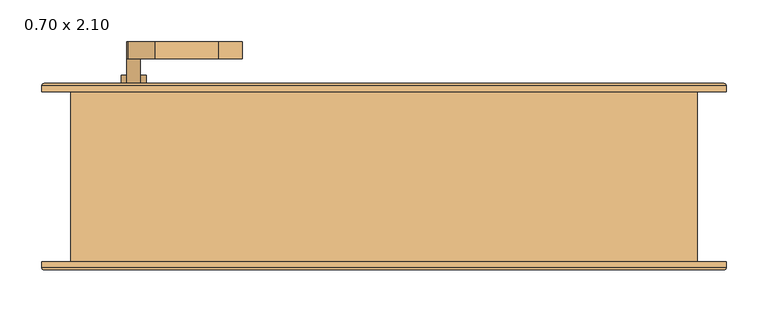
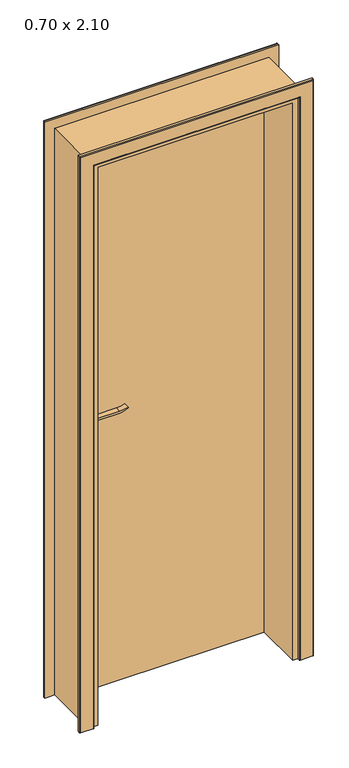
"""IFC4 building model written with IfcOpenShell, lengths in millimetres: door geometry, .CC_ND 300_PORTA SIMPLES DE ABRIR_COM EXTENSÃO : 0.70 x 2.10."""

from ifc_helpers import new_model, si_unit, point, frame, frame_2d, origin, origin_with_axes, place, context, project, spatial, polyline, circle_curve, ellipse_curve, trimmed, segment, composite_curve, outline, extrude, faceted_brep, source, transform, mapped, element, save
from ifc_brep_helpers import plane_surface, cylinder_surface, advanced_brep


def door_0_70_x_2_10_fae9ef36(model_context):
    return source(origin(), model_context, "Body", "SolidModel", [
        extrude(outline(composite_curve([segment(trimmed(circle_curve(frame_2d((964.5, -300.0)), 15.0), [point((964.5, -285.0))], [point((964.5, -315.0))], False, "CARTESIAN"), True, "CONTINUOUS"), segment(trimmed(circle_curve(frame_2d((964.5, -300.0)), 15.0), [point((964.5, -315.0))], [point((964.5, -285.0))], False, "CARTESIAN"), True, "CONTINUOUS")], self_intersect=False)), frame((0.0, 126.4, 0.0), z_axis=(0.0, 1.0, 0.0), x_axis=(0.0, 0.0, 1.0)), (0.0, 0.0, 1.0), 10.0),
        extrude(outline(composite_curve([segment(trimmed(circle_curve(frame_2d((964.5, -300.0)), 15.0), [point((964.5, -285.0))], [point((964.5, -315.0))], False, "CARTESIAN"), True, "CONTINUOUS"), segment(trimmed(circle_curve(frame_2d((964.5, -300.0)), 15.0), [point((964.5, -315.0))], [point((964.5, -285.0))], False, "CARTESIAN"), True, "CONTINUOUS")], self_intersect=False)), frame((0.0, 66.4, 0.0), z_axis=(0.0, 1.0, 0.0), x_axis=(0.0, 0.0, 1.0)), (0.0, 0.0, 1.0), 10.0),
        extrude(outline(composite_curve([segment(trimmed(circle_curve(frame_2d((1024.5, -300.0)), 8.0), [point((1029.1523287, -306.5081363))], [point((1024.5, -292.0))], False, "CARTESIAN"), True, "CONTINUOUS"), segment(trimmed(circle_curve(frame_2d((1019.3738613, -274.6138099)), 18.1261387), [point((1024.5, -292.0))], [point((1037.5, -274.6138099))], True, "CARTESIAN"), True, "CONTINUOUS"), segment(polyline([(1037.5, -274.6138099), (1037.5, -198.3564091)]), True, "CONTINUOUS"), segment(trimmed(circle_curve(frame_2d((1096.7709207, -201.9396612)), 59.3791355), [point((1037.5, -198.3564091))], [point((1046.7135558, -170.0))], False, "CARTESIAN"), True, "CONTINUOUS"), segment(polyline([(1046.7135558, -170.0), (1049.5, -170.0)]), True, "CONTINUOUS"), segment(trimmed(circle_curve(frame_2d((1127.7850638, -198.4227909)), 83.2850902), [point((1049.5, -170.0))], [point((1044.5, -198.3564091))], True, "CARTESIAN"), True, "CONTINUOUS"), segment(polyline([(1044.5, -198.3564091), (1044.5, -274.6325667)]), True, "CONTINUOUS"), segment(trimmed(circle_curve(frame_2d((1007.2555521, -276.3324871)), 37.2832219), [point((1044.5, -274.6325667))], [point((1029.1523287, -306.5081363))], False, "CARTESIAN"), True, "CONTINUOUS")], self_intersect=False)), frame((0.0, 156.4, 0.0), z_axis=(0.0, 1.0, 0.0), x_axis=(0.0, 0.0, 1.0)), (0.0, 0.0, 1.0), 20.0),
        extrude(outline(composite_curve([segment(trimmed(circle_curve(frame_2d((1019.3738682, -274.6138122)), 18.1261318), [point((1024.4999903, -292.0))], [point((1037.5, -274.6138122))], True, "CARTESIAN"), True, "CONTINUOUS"), segment(polyline([(1037.5, -274.6138122), (1037.5, -198.3564091)]), True, "CONTINUOUS"), segment(trimmed(circle_curve(frame_2d((1096.7709207, -201.9396612)), 59.3791355), [point((1037.5, -198.3564091))], [point((1046.7135558, -170.0))], False, "CARTESIAN"), True, "CONTINUOUS"), segment(polyline([(1046.7135558, -170.0), (1049.5, -170.0)]), True, "CONTINUOUS"), segment(trimmed(circle_curve(frame_2d((1127.7850638, -198.4227909)), 83.2850902), [point((1049.5, -170.0))], [point((1044.5, -198.3564091))], True, "CARTESIAN"), True, "CONTINUOUS"), segment(polyline([(1044.5, -198.3564091), (1044.5, -274.6325667)]), True, "CONTINUOUS"), segment(trimmed(circle_curve(frame_2d((1007.2555521, -276.3324871)), 37.2832219), [point((1044.5, -274.6325667))], [point((1029.1523287, -306.5081363))], False, "CARTESIAN"), True, "CONTINUOUS"), segment(trimmed(circle_curve(frame_2d((1024.5, -300.0)), 8.0), [point((1029.1523287, -306.5081363))], [point((1024.4999903, -292.0))], False, "CARTESIAN"), True, "CONTINUOUS")], self_intersect=False)), frame((0.0, 26.4, 0.0), z_axis=(0.0, 1.0, 0.0), x_axis=(0.0, 0.0, 1.0)), (0.0, 0.0, 1.0), 20.0),
        extrude(outline(composite_curve([segment(trimmed(circle_curve(frame_2d((1024.5, -300.0)), 8.0), [point((1024.5, -292.0))], [point((1024.5, -308.0))], False, "CARTESIAN"), True, "CONTINUOUS"), segment(trimmed(circle_curve(frame_2d((1024.5, -300.0)), 8.0), [point((1024.5, -308.0))], [point((1024.5, -292.0))], False, "CARTESIAN"), True, "CONTINUOUS")], self_intersect=False)), frame((0.0, 126.4, 0.0), z_axis=(0.0, 1.0, 0.0), x_axis=(0.0, 0.0, 1.0)), (0.0, 0.0, 1.0), 30.0),
        extrude(outline(composite_curve([segment(trimmed(circle_curve(frame_2d((1024.5, -300.0)), 8.0), [point((1024.5, -292.0))], [point((1024.5, -308.0))], False, "CARTESIAN"), True, "CONTINUOUS"), segment(trimmed(circle_curve(frame_2d((1024.5, -300.0)), 8.0), [point((1024.5, -308.0))], [point((1024.5, -292.0))], False, "CARTESIAN"), True, "CONTINUOUS")], self_intersect=False)), frame((0.0, 46.4, 0.0), z_axis=(0.0, 1.0, 0.0), x_axis=(0.0, 0.0, 1.0)), (0.0, 0.0, 1.0), 30.0),
        extrude(outline(composite_curve([segment(trimmed(circle_curve(frame_2d((954.5, -300.0)), 25.0), [point((954.5, -325.0))], [point((954.5, -275.0))], False, "CARTESIAN"), True, "CONTINUOUS"), segment(polyline([(954.5, -275.0), (1024.5, -275.0)]), True, "CONTINUOUS"), segment(trimmed(circle_curve(frame_2d((1024.5, -300.0)), 25.0), [point((1024.5, -275.0))], [point((1024.5, -325.0))], False, "CARTESIAN"), True, "CONTINUOUS"), segment(polyline([(1024.5, -325.0), (954.5, -325.0)]), True, "CONTINUOUS")], self_intersect=False)), frame((0.0, 116.4, 0.0), z_axis=(0.0, 1.0, 0.0), x_axis=(0.0, 0.0, 1.0)), (0.0, 0.0, 1.0), 10.0),
        extrude(outline(composite_curve([segment(trimmed(circle_curve(frame_2d((954.5, -300.0)), 25.0), [point((954.5, -325.0))], [point((954.5, -275.0))], False, "CARTESIAN"), True, "CONTINUOUS"), segment(polyline([(954.5, -275.0), (1024.5, -275.0)]), True, "CONTINUOUS"), segment(trimmed(circle_curve(frame_2d((1024.5, -300.0)), 25.0), [point((1024.5, -275.0))], [point((1024.5, -325.0))], False, "CARTESIAN"), True, "CONTINUOUS"), segment(polyline([(1024.5, -325.0), (954.5, -325.0)]), True, "CONTINUOUS")], self_intersect=False)), frame((0.0, 76.4, 0.0), z_axis=(0.0, 1.0, 0.0), x_axis=(0.0, 0.0, 1.0)), (0.0, 0.0, 1.0), 10.0),
        faceted_brep([(342.0, -86.9, 0.0), (342.0, 86.4, 0.0), (350.0, 86.4, 0.0), (350.0, 116.4, 0.0), (375.0, 116.4, 0.0), (375.0, -86.9, 0.0), (375.0, -86.9, 2100.0), (-375.0, -86.9, 2100.0), (-375.0, -86.9, 0.0), (-342.0, -86.9, 0.0), (-342.0, -86.9, 2067.0), (342.0, -86.9, 2067.0), (375.0, 116.4, 2100.0), (350.0, 116.4, 2075.0), (-350.0, 116.4, 2075.0), (-350.0, 116.4, 0.0), (-375.0, 116.4, 0.0), (-375.0, 116.4, 2100.0), (350.0, 86.4, 2075.0), (342.0, 86.4, 2067.0), (-342.0, 86.4, 2067.0), (-342.0, 86.4, 0.0), (-350.0, 86.4, 0.0), (-350.0, 86.4, 2075.0)], [[[0, 1, 2, 3, 4, 5]], [[5, 6, 7, 8, 9, 10, 11, 0]], [[4, 12, 6, 5]], [[3, 13, 14, 15, 16, 17, 12, 4]], [[2, 18, 13, 3]], [[1, 19, 20, 21, 22, 23, 18, 2]], [[0, 11, 19, 1]], [[10, 9, 21, 20]], [[9, 8, 16, 15, 22, 21]], [[17, 16, 8, 7]], [[23, 22, 15, 14]], [[12, 17, 7, 6]], [[18, 23, 14, 13]], [[11, 10, 20, 19]]]),
        extrude(outline(polyline([(-350.0, 86.4), (-350.0, 116.4), (350.0, 116.4), (350.0, 86.4), (-350.0, 86.4)])), origin_with_axes(), (0.0, 0.0, 1.0), 2075.0),
        advanced_brep(
        [(-410.0, 116.4, 0.0), (-410.0, 123.4, 0.0), (-407.0, 126.4, 0.0), (-363.0, 126.4, 0.0), (-360.0, 123.4, 0.0), (-360.0, 116.4, 0.0), (-360.0, 116.4, 2085.0), (360.0, 116.4, 2085.0), (360.0, 116.4, 0.0), (410.0, 116.4, 0.0), (410.0, 116.4, 2135.0), (-410.0, 116.4, 2135.0), (-360.0, 123.4, 2085.0), (-363.0, 126.4, 2088.0), (-407.0, 126.4, 2132.0), (407.0, 126.4, 2132.0), (407.0, 126.4, 0.0), (363.0, 126.4, 0.0), (363.0, 126.4, 2088.0), (-410.0, 123.4, 2135.0), (410.0, 123.4, 0.0), (410.0, 123.4, 2135.0), (360.0, 123.4, 0.0), (360.0, 123.4, 2085.0)],
        [
            (0, 1),
            (1, 2, circle_curve(frame((-407.0, 123.4, 0.0), z_axis=(0.0, 0.0, -1.0), x_axis=(1.0, 0.0, 0.0)), 3.0)),
            (2, 3),
            (3, 4, circle_curve(frame((-363.0, 123.4, 0.0), z_axis=(0.0, 0.0, -1.0), x_axis=(1.0, 0.0, 0.0)), 3.0)),
            (4, 5),
            (5, 0),
            (5, 6),
            (6, 7),
            (7, 8),
            (8, 9),
            (9, 10),
            (10, 11),
            (11, 0),
            (4, 12),
            (12, 6),
            (3, 13),
            (13, 12, ellipse_curve(frame((-363.0, 123.4, 2088.0), z_axis=(-0.7071067811865475, 0.0, -0.7071067811865475), x_axis=(0.7071067811865474, 0.0, -0.7071067811865476)), 4.2426407, 3.0)),
            (2, 14),
            (14, 15),
            (15, 16),
            (16, 17),
            (17, 18),
            (18, 13),
            (1, 19),
            (19, 14, ellipse_curve(frame((-407.0, 123.4, 2132.0), z_axis=(-0.7071067811865475, 0.0, -0.7071067811865475), x_axis=(0.7071067811865474, 0.0, -0.7071067811865476)), 4.2426407, 3.0)),
            (11, 19),
            (9, 20),
            (20, 21),
            (21, 10),
            (8, 22),
            (22, 17, circle_curve(frame((363.0, 123.4, 0.0), z_axis=(0.0, 0.0, -1.0), x_axis=(-1.0, 0.0, 0.0)), 3.0)),
            (16, 20, circle_curve(frame((407.0, 123.4, 0.0), z_axis=(0.0, 0.0, -1.0), x_axis=(-1.0, 0.0, 0.0)), 3.0)),
            (23, 22),
            (7, 23),
            (23, 18, ellipse_curve(frame((363.0, 123.4, 2088.0), z_axis=(0.7071067811865475, 0.0, -0.7071067811865475), x_axis=(0.7071067811865474, 0.0, 0.7071067811865476)), 4.2426407, 3.0)),
            (15, 21, ellipse_curve(frame((407.0, 123.4, 2132.0), z_axis=(0.7071067811865475, 0.0, -0.7071067811865475), x_axis=(0.7071067811865474, 0.0, 0.7071067811865476)), 4.2426407, 3.0)),
            (12, 23),
            (21, 19),
        ],
        [
            plane_surface(frame((-360.0, 116.4, 0.0), z_axis=(0.0, 0.0, -1.0), x_axis=(0.0, -1.0, 0.0))),
            plane_surface(frame((-410.0, 116.4, 0.0), z_axis=(0.0, -1.0, 0.0), x_axis=(0.0, 0.0, 1.0))),
            plane_surface(frame((-360.0, 116.4, 0.0), z_axis=(1.0, 0.0, 0.0), x_axis=(0.0, 0.0, 1.0))),
            cylinder_surface(frame((-363.0, 123.4, 0.0), z_axis=(0.0, 0.0, -1.0), x_axis=(1.0, 0.0, 0.0)), 3.0),
            plane_surface(frame((-363.0, 126.4, 0.0), z_axis=(0.0, 1.0, 0.0), x_axis=(0.0, 0.0, 1.0))),
            cylinder_surface(frame((-407.0, 123.4, 0.0), z_axis=(0.0, 0.0, -1.0), x_axis=(1.0, 0.0, 0.0)), 3.0),
            plane_surface(frame((-410.0, 123.4, 0.0), z_axis=(-1.0, 0.0, 0.0), x_axis=(0.0, 0.0, 1.0))),
            plane_surface(frame((410.0, 123.4, 2135.0), z_axis=(1.0, 0.0, 0.0), x_axis=(0.0, 0.0, -1.0))),
            plane_surface(frame((360.0, 116.4, 0.0), z_axis=(0.0, 0.0, -1.0), x_axis=(0.0, -1.0, 0.0))),
            plane_surface(frame((360.0, 116.4, 2085.0), z_axis=(-1.0, 0.0, 0.0), x_axis=(0.0, 0.0, -1.0))),
            cylinder_surface(frame((363.0, 123.4, 2085.0), z_axis=(0.0, 0.0, 1.0), x_axis=(-1.0, 0.0, 0.0)), 3.0),
            cylinder_surface(frame((407.0, 123.4, 2085.0), z_axis=(0.0, 0.0, 1.0), x_axis=(-1.0, 0.0, 0.0)), 3.0),
            plane_surface(frame((-360.0, 116.4, 2085.0), z_axis=(0.0, 0.0, -1.0), x_axis=(1.0, 0.0, 0.0))),
            plane_surface(frame((-410.0, 123.4, 2135.0), z_axis=(0.0, 0.0, 1.0), x_axis=(1.0, 0.0, 0.0))),
            cylinder_surface(frame((-360.0, 123.4, 2088.0), z_axis=(-1.0, 0.0, 0.0), x_axis=(0.0, 0.0, -1.0)), 3.0),
            cylinder_surface(frame((-360.0, 123.4, 2132.0), z_axis=(-1.0, 0.0, 0.0), x_axis=(0.0, 0.0, -1.0)), 3.0),
        ],
        [
            (0, [[1, 2, 3, 4, 5, 6]]),
            (1, [[7, 8, 9, 10, 11, 12, 13, -6]]),
            (2, [[14, 15, -7, -5]]),
            (3, [[16, 17, -14, -4]]),
            (4, [[18, 19, 20, 21, 22, 23, -16, -3]]),
            (5, [[24, 25, -18, -2]]),
            (6, [[-13, 26, -24, -1]]),
            (7, [[-11, 27, 28, 29]]),
            (8, [[-10, 30, 31, -21, 32, -27]]),
            (9, [[33, -30, -9, 34]]),
            (10, [[-22, -31, -33, 35]]),
            (11, [[-28, -32, -20, 36]]),
            (12, [[37, -34, -8, -15]]),
            (13, [[-12, -29, 38, -26]]),
            (14, [[-23, -35, -37, -17]]),
            (15, [[-38, -36, -19, -25]]),
        ],
    ),
        advanced_brep(
        [(410.0, -86.9, 0.0), (410.0, -93.9342217, 0.0), (407.0342217, -96.9, 0.0), (362.9842717, -96.9, 0.0), (360.0, -93.9157283, 0.0), (360.0, -86.9, 0.0), (360.0, -86.9, 2085.0), (-360.0, -86.9, 2085.0), (-360.0, -86.9, 0.0), (-410.0, -86.9, 0.0), (-410.0, -86.9, 2135.0), (410.0, -86.9, 2135.0), (360.0, -93.9157283, 2085.0), (362.9842717, -96.9, 2087.9842717), (407.0342217, -96.9, 2132.0342217), (-407.0342217, -96.9, 2132.0342217), (-407.0342217, -96.9, 0.0), (-362.9842717, -96.9, 0.0), (-362.9842717, -96.9, 2087.9842717), (410.0, -93.9342217, 2135.0), (-410.0, -93.9342217, 0.0), (-410.0, -93.9342217, 2135.0), (-360.0, -93.9157283, 0.0), (-360.0, -93.9157283, 2085.0)],
        [
            (0, 1),
            (1, 2, circle_curve(frame((407.0342217, -93.9342217, 0.0), z_axis=(0.0, 0.0, -1.0), x_axis=(1.0, 0.0, 0.0)), 2.9657783)),
            (2, 3),
            (3, 4, circle_curve(frame((362.9842717, -93.9157283, 0.0), z_axis=(0.0, 0.0, -1.0), x_axis=(1.0, 0.0, 0.0)), 2.9842717)),
            (4, 5),
            (5, 0),
            (5, 6),
            (6, 7),
            (7, 8),
            (8, 9),
            (9, 10),
            (10, 11),
            (11, 0),
            (4, 12),
            (12, 6),
            (3, 13),
            (13, 12, ellipse_curve(frame((362.9842717, -93.9157283, 2087.9842717), z_axis=(0.7071067811865475, 0.0, -0.7071067811865475), x_axis=(-0.7071067811865474, 0.0, -0.7071067811865476)), 4.2203975, 2.9842717)),
            (2, 14),
            (14, 15),
            (15, 16),
            (16, 17),
            (17, 18),
            (18, 13),
            (1, 19),
            (19, 14, ellipse_curve(frame((407.0342217, -93.9342217, 2132.0342217), z_axis=(0.7071067811865475, 0.0, -0.7071067811865475), x_axis=(-0.7071067811865474, 0.0, -0.7071067811865476)), 4.1942438, 2.9657783)),
            (11, 19),
            (9, 20),
            (20, 21),
            (21, 10),
            (8, 22),
            (22, 17, circle_curve(frame((-362.9842717, -93.9157283, 0.0), z_axis=(0.0, 0.0, -1.0), x_axis=(-1.0, 0.0, 0.0)), 2.9842717)),
            (16, 20, circle_curve(frame((-407.0342217, -93.9342217, 0.0), z_axis=(0.0, 0.0, -1.0), x_axis=(-1.0, 0.0, 0.0)), 2.9657783)),
            (23, 22),
            (7, 23),
            (23, 18, ellipse_curve(frame((-362.9842717, -93.9157283, 2087.9842717), z_axis=(-0.7071067811865475, 0.0, -0.7071067811865475), x_axis=(-0.7071067811865474, 0.0, 0.7071067811865476)), 4.2203975, 2.9842717)),
            (15, 21, ellipse_curve(frame((-407.0342217, -93.9342217, 2132.0342217), z_axis=(-0.7071067811865475, 0.0, -0.7071067811865475), x_axis=(-0.7071067811865474, 0.0, 0.7071067811865476)), 4.1942438, 2.9657783)),
            (12, 23),
            (21, 19),
        ],
        [
            plane_surface(frame((360.0, -86.9, 0.0), z_axis=(0.0, 0.0, -1.0), x_axis=(0.0, -1.0, 0.0))),
            plane_surface(frame((410.0, -86.9, 0.0), z_axis=(0.0, 1.0, 0.0), x_axis=(0.0, 0.0, 1.0))),
            plane_surface(frame((360.0, -86.9, 0.0), z_axis=(-1.0, 0.0, 0.0), x_axis=(0.0, 0.0, 1.0))),
            cylinder_surface(frame((362.9842717, -93.9157283, 0.0), z_axis=(0.0, 0.0, -1.0), x_axis=(1.0, 0.0, 0.0)), 2.9842717),
            plane_surface(frame((362.9842717, -96.9, 0.0), z_axis=(0.0, -1.0, 0.0), x_axis=(0.0, 0.0, 1.0))),
            cylinder_surface(frame((407.0342217, -93.9342217, 0.0), z_axis=(0.0, 0.0, -1.0), x_axis=(1.0, 0.0, 0.0)), 2.9657783),
            plane_surface(frame((410.0, -93.9342217, 0.0), z_axis=(1.0, 0.0, 0.0), x_axis=(0.0, 0.0, 1.0))),
            plane_surface(frame((-410.0, -93.9342217, 2135.0), z_axis=(-1.0, 0.0, 0.0), x_axis=(0.0, 0.0, -1.0))),
            plane_surface(frame((-360.0, -86.9, 0.0), z_axis=(0.0, 0.0, -1.0), x_axis=(0.0, -1.0, 0.0))),
            plane_surface(frame((-360.0, -86.9, 2085.0), z_axis=(1.0, 0.0, 0.0), x_axis=(0.0, 0.0, -1.0))),
            cylinder_surface(frame((-362.9842717, -93.9157283, 2085.0), z_axis=(0.0, 0.0, 1.0), x_axis=(-1.0, 0.0, 0.0)), 2.9842717),
            cylinder_surface(frame((-407.0342217, -93.9342217, 2085.0), z_axis=(0.0, 0.0, 1.0), x_axis=(-1.0, 0.0, 0.0)), 2.9657783),
            plane_surface(frame((360.0, -86.9, 2085.0), z_axis=(0.0, 0.0, -1.0), x_axis=(-1.0, 0.0, 0.0))),
            plane_surface(frame((410.0, -93.9342217, 2135.0), z_axis=(0.0, 0.0, 1.0), x_axis=(-1.0, 0.0, 0.0))),
            cylinder_surface(frame((360.0, -93.9157283, 2087.9842717), z_axis=(1.0, 0.0, 0.0), x_axis=(0.0, 0.0, 1.0)), 2.9842717),
            cylinder_surface(frame((360.0, -93.9342217, 2132.0342217), z_axis=(1.0, 0.0, 0.0), x_axis=(0.0, 0.0, 1.0)), 2.9657783),
        ],
        [
            (0, [[1, 2, 3, 4, 5, 6]]),
            (1, [[7, 8, 9, 10, 11, 12, 13, -6]]),
            (2, [[14, 15, -7, -5]]),
            (3, [[16, 17, -14, -4]]),
            (4, [[18, 19, 20, 21, 22, 23, -16, -3]]),
            (5, [[24, 25, -18, -2]]),
            (6, [[-13, 26, -24, -1]]),
            (7, [[-11, 27, 28, 29]]),
            (8, [[-10, 30, 31, -21, 32, -27]]),
            (9, [[33, -30, -9, 34]]),
            (10, [[-22, -31, -33, 35]]),
            (11, [[-28, -32, -20, 36]]),
            (12, [[37, -34, -8, -15]]),
            (13, [[-12, -29, 38, -26]]),
            (14, [[-23, -35, -37, -17]]),
            (15, [[-38, -36, -19, -25]]),
        ],
    ),
    ])


if __name__ == "__main__":
    model = new_model("IFC4")
    model_context = context("Model", 3, world=origin())
    ifc_project = project(units=[si_unit("LENGTHUNIT", "METRE", prefix="MILLI")], contexts=[model_context])
    site = spatial("IfcSite", under=ifc_project)
    building = spatial("IfcBuilding", under=site)
    placement = place(None, origin())
    door_0_70_x_2_10_shape = door_0_70_x_2_10_fae9ef36(model_context)
    element("IfcDoor", 1, ObjectType=".CC_ND 300_PORTA SIMPLES DE ABRIR_COM EXTENSÃO : 0.70 x 2.10", at=placement, inside=building, context=model_context, shape_type="MappedRepresentation", body=[
        mapped(door_0_70_x_2_10_shape, transform((0.0, 0.0, 0.0), x_axis=(1.0, 0.0, 0.0), y_axis=(0.0, 1.0, 0.0), z_axis=(0.0, 0.0, 1.0))),
    ])
    save(model, "model.ifc")

# Revit data of these elements
# Type ".CC_ND 300_PORTA SIMPLES DE ABRIR_COM EXTENSÃO : 0.70 x 2.10"
#   Type Mark = "155"
#   Analytic Construction = "<None>"
#   Rough Width = 0.75 m
#   Espessura moldura externa = 0.01 m
#   Espessura moldura interna = 0.01 m
#   Largura moldura = 0.05 m
#   Extensão acabamento exterior [instance default] = 0.00 m
#   Extensão acabamento interior [instance default] = 0.00 m
#   Espessura batente = 0.025 m
#   Thickness = 0.03 m
#   Altura batente = 2.085 m
#   Aux Arco [instance default] = 0.70 m
#   Rough Height = 2.125 m
#   Height = 2.10 m
#   Width = 0.70 m
#   Moldura interna [instance default] = yes
#   Moldura externa [instance default] = yes
#   Porta = .MADEIRA COM PINTURA ESMALTE BRANCO ACETINADO
#   Moldura = .MADEIRA COM PINTURA ESMALTE BRANCO ACETINADO
#   Maçaneta = .ALUMÍNIO
#   Batente = .MADEIRA COM PINTURA ESMALTE BRANCO ACETINADO
#   Function = (empty or 0)
#   Wall Closure = (empty or 0)
# Element 1 (IfcDoor, ".CC_ND 300_PORTA SIMPLES DE ABRIR_COM EXTENSÃO : 0.70 x 2.10")
#   Extensão acabamento interior = 0.0295 m
#   Aux Arco = 0.7295 m
#   Materials on its faces: ".MADEIRA COM PINTURA ESMALTE BRANCO ACETINADO", ".ALUMÍNIO"
# Materials
#   ".MADEIRA COM PINTURA ESMALTE BRANCO ACETINADO": class ".CC_MADEIRAS", colour RGB 240 240 240, transparency 0, Description = "Madeira com pintura esmalte branco acetinado.", Cost = 0
#   ".ALUMÍNIO": class "CC_METAIS", colour RGB 244 244 244, transparency 0, Description = "Material alumínio", Cost = 0
